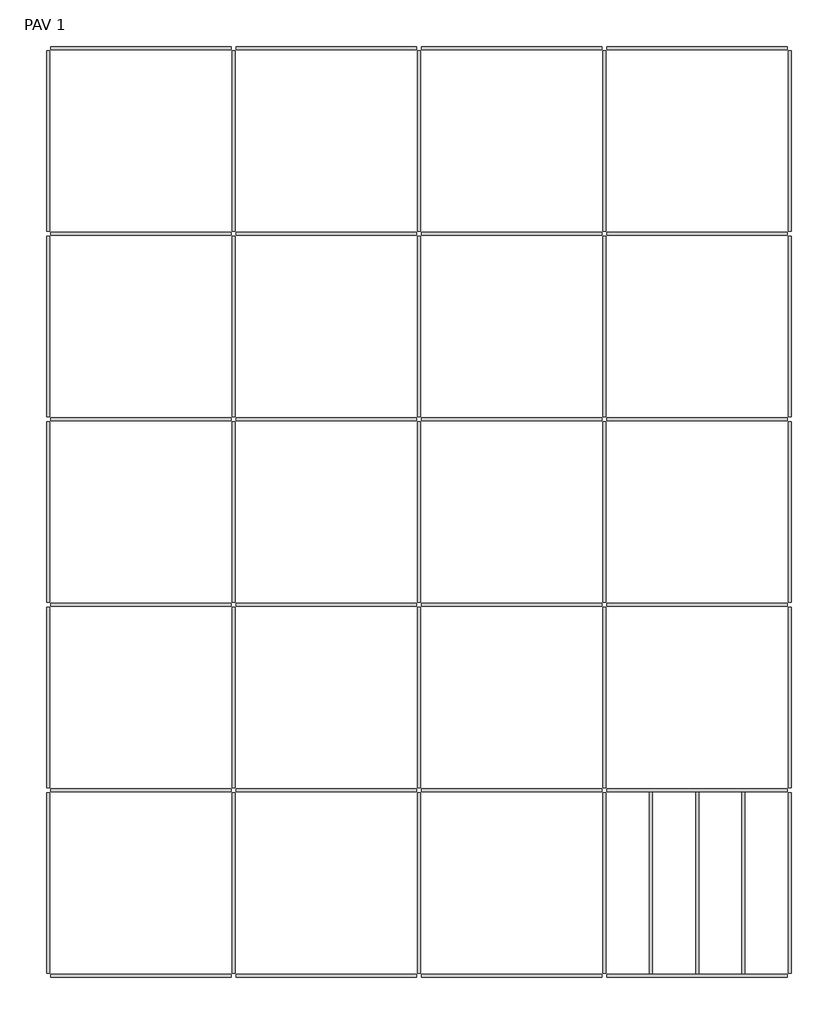
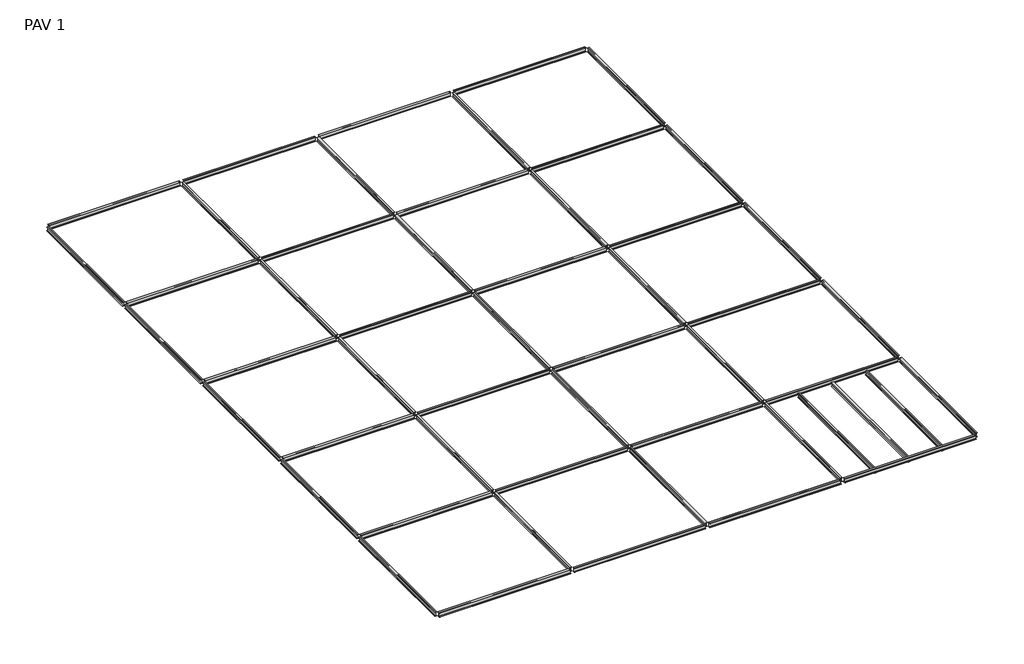
# One storey: 52 beams.
"""IFC4 building model written with IfcOpenShell, lengths in millimetres."""

import ifcopenshell
import ifcopenshell.guid

model = None  # the IFC model being written
_history = None  # IfcOwnerHistory: only IFC2X3 demands one
_inside = {}  # id of a spatial element -> (the spatial element, [elements in it])
_under = {}  # id of a project, library or spatial element -> (it, [spatial elements below it])
_declared = {}  # id of a project -> (the project, [libraries it declares])
_typed = {}  # id of a type object -> (the type object, [elements of that type])
_made_of = {}  # id of a material, layer set ... -> (it, [elements and type objects made of it])


def new_model(schema):
    """Start an empty IFC model of exactly this schema.

    Asked for "IFC4X3", IfcOpenShell would pick the latest addendum, in which some entities
    have other attributes; the version numbers below select the first issue.
    IFC2X3 requires an IfcOwnerHistory on every rooted entity: one is made here for all.
    """
    global model, _history
    if schema == "IFC4X3":
        model = ifcopenshell.file(schema_version=(4, 3, 0, 0))
    else:
        model = ifcopenshell.file(schema=schema)
    _inside.clear()
    _under.clear()
    _declared.clear()
    _typed.clear()
    _made_of.clear()
    _history = None
    if model.schema == "IFC2X3":
        org = make("IfcOrganization", Name="unknown")
        user = make(
            "IfcPersonAndOrganization",
            ThePerson=make("IfcPerson", FamilyName="unknown"),
            TheOrganization=org,
        )
        app = make(
            "IfcApplication",
            ApplicationDeveloper=org,
            Version="unknown",
            ApplicationFullName="unknown",
            ApplicationIdentifier="unknown",
        )
        _history = make(
            "IfcOwnerHistory",
            OwningUser=user,
            OwningApplication=app,
            ChangeAction="ADDED",
            CreationDate=0,
        )
    return model


def make(cls, **values):
    """One entity of the class cls with the attributes given. An attribute that is None is left unset."""
    return model.create_entity(
        cls, **{name: value for name, value in values.items() if value is not None}
    )


def rooted(cls, **values):
    """An entity with a GlobalId (a new one), such as an element, a storey or a relation."""
    return make(cls, GlobalId=ifcopenshell.guid.new(), OwnerHistory=_history, **values)


def si_unit(unit_type, name, prefix=None):
    """IfcSIUnit, for example si_unit("LENGTHUNIT", "METRE", prefix="MILLI")."""
    return make("IfcSIUnit", UnitType=unit_type, Prefix=prefix, Name=name)


def assignment(units):
    """IfcUnitAssignment: the units of a project."""
    return None if units is None else make("IfcUnitAssignment", Units=units)


def point(xyz):
    """IfcCartesianPoint."""
    return None if xyz is None else make("IfcCartesianPoint", Coordinates=xyz)


def direction(xyz):
    """IfcDirection."""
    return None if xyz is None else make("IfcDirection", DirectionRatios=xyz)


def frame(location, z_axis=None, x_axis=None):
    """IfcAxis2Placement3D, a coordinate frame: its origin and axes. An axis left out is left unset."""
    return make(
        "IfcAxis2Placement3D",
        Location=point(location),
        Axis=direction(z_axis),
        RefDirection=direction(x_axis),
    )


def frame_2d(location, x_axis=None):
    """IfcAxis2Placement2D, a coordinate frame in the plane: its origin and x axis."""
    return make(
        "IfcAxis2Placement2D", Location=point(location), RefDirection=direction(x_axis)
    )


def origin():
    """The frame at (0, 0, 0) with its axes left unset."""
    return frame((0.0, 0.0, 0.0))


def place(relative_to, where):
    """IfcLocalPlacement: puts the frame where relative to a parent placement (None: the world)."""
    return make(
        "IfcLocalPlacement", PlacementRelTo=relative_to, RelativePlacement=where
    )


def context(
    kind, dimensions, precision=None, world=None, true_north=None, identifier=None
):
    """IfcGeometricRepresentationContext, for example the 3D "Model" context."""
    return make(
        "IfcGeometricRepresentationContext",
        ContextIdentifier=identifier,
        ContextType=kind,
        CoordinateSpaceDimension=dimensions,
        Precision=precision,
        WorldCoordinateSystem=world,
        TrueNorth=true_north,
    )


def project(units=None, contexts=None):
    """IfcProject with its units and contexts."""
    return rooted(
        "IfcProject",
        Name="project",
        RepresentationContexts=contexts,
        UnitsInContext=assignment(units),
    )


def spatial(cls, under=None, at=None, **own):
    """A site, building, storey or space (cls), placed at a placement, below another one or the project."""
    s = rooted(cls, ObjectPlacement=at, **own)
    if under is not None:
        _under.setdefault(under.id(), (under, []))[1].append(s)
    return s


def polyline(points):
    """IfcPolyline through the points."""
    return make("IfcPolyline", Points=[point(p) for p in points])


def circle_curve(where, radius):
    """IfcCircle in the frame where."""
    return make("IfcCircle", Position=where, Radius=radius)


def trimmed(basis, trim1, trim2, sense, master):
    """IfcTrimmedCurve: the piece of a basis curve between two trims."""
    return make(
        "IfcTrimmedCurve",
        BasisCurve=basis,
        Trim1=trim1,
        Trim2=trim2,
        SenseAgreement=sense,
        MasterRepresentation=master,
    )


def segment(curve, same_sense, transition):
    """IfcCompositeCurveSegment."""
    return make(
        "IfcCompositeCurveSegment",
        Transition=transition,
        SameSense=same_sense,
        ParentCurve=curve,
    )


def composite_curve(segments, self_intersect=None):
    """IfcCompositeCurve: segments joined end to end."""
    return make("IfcCompositeCurve", Segments=segments, SelfIntersect=self_intersect)


def outline(outer, holes=None, kind="AREA"):
    """IfcArbitraryClosedProfileDef: a profile drawn as a closed curve; with holes, ...WithVoids."""
    if holes is None:
        return make("IfcArbitraryClosedProfileDef", ProfileType=kind, OuterCurve=outer)
    return make(
        "IfcArbitraryProfileDefWithVoids",
        ProfileType=kind,
        OuterCurve=outer,
        InnerCurves=holes,
    )


def extrude(swept, where, along, depth):
    """IfcExtrudedAreaSolid: the profile swept, set in the frame where, extruded along a direction by depth."""
    return make(
        "IfcExtrudedAreaSolid",
        SweptArea=swept,
        Position=where,
        ExtrudedDirection=direction(along),
        Depth=depth,
    )


def shape(context_of_items, identifier, shape_type, items):
    """IfcShapeRepresentation: the items that make up one representation, for example the "Body"."""
    return make(
        "IfcShapeRepresentation",
        ContextOfItems=context_of_items,
        RepresentationIdentifier=identifier,
        RepresentationType=shape_type,
        Items=items,
    )


def source(mapping_origin, context_of_items, identifier, shape_type, items):
    """IfcRepresentationMap: a shape defined once, which mapped items show again and again."""
    return make(
        "IfcRepresentationMap",
        MappingOrigin=mapping_origin,
        MappedRepresentation=shape(context_of_items, identifier, shape_type, items),
    )


def transform(
    local_origin,
    x_axis=None,
    y_axis=None,
    z_axis=None,
    scale=None,
    scale2=None,
    scale3=None,
    uniform=True,
):
    """IfcCartesianTransformationOperator3D, or its non-uniform kind. x_axis, y_axis, z_axis: its Axis1, 2, 3."""
    if uniform:
        return make(
            "IfcCartesianTransformationOperator3D",
            Axis1=direction(x_axis),
            Axis2=direction(y_axis),
            LocalOrigin=point(local_origin),
            Scale=scale,
            Axis3=direction(z_axis),
        )
    return make(
        "IfcCartesianTransformationOperator3DnonUniform",
        Axis1=direction(x_axis),
        Axis2=direction(y_axis),
        LocalOrigin=point(local_origin),
        Scale=scale,
        Axis3=direction(z_axis),
        Scale2=scale2,
        Scale3=scale3,
    )


def mapped(mapping_source, mapping_target):
    """IfcMappedItem: shows the shape of a source again, moved by a transform."""
    return make(
        "IfcMappedItem", MappingSource=mapping_source, MappingTarget=mapping_target
    )


def made_of(thing, what):
    """Note that an element or type object is made of a material, layer set ...; save() writes the relation."""
    if what is not None:
        _made_of.setdefault(what.id(), (what, []))[1].append(thing)
    return thing


def element(
    cls,
    number,
    at=None,
    inside=None,
    cuts=None,
    type_object=None,
    material=None,
    context=None,
    identifier="Body",
    shape_type=None,
    held_by="IfcProductDefinitionShape",
    body=None,
    shapes=None,
    **own,
):
    """One element of the class cls, such as IfcWall. Its Tag is "e" and its number.

    at: its placement. inside: the storey or other place that contains it. cuts: it is an
    opening in that element (IfcRelVoidsElement). A single representation is given by context,
    identifier, shape_type and body (its items); several are given by shapes. held_by: the class
    of the entity that holds the representations. save() writes the other relations.
    """
    e = rooted(cls, Tag="e%d" % number, ObjectPlacement=at, **own)
    if body is not None:
        shapes = [shape(context, identifier, shape_type, body)]
    if shapes is not None:
        e.Representation = make(held_by, Representations=shapes)
    if inside is not None:
        _inside.setdefault(inside.id(), (inside, []))[1].append(e)
    if cuts is not None:
        rooted(
            "IfcRelVoidsElement", RelatingBuildingElement=cuts, RelatedOpeningElement=e
        )
    if type_object is not None:
        _typed.setdefault(type_object.id(), (type_object, []))[1].append(e)
    return made_of(e, material)


def aggregate(whole, parts):
    """IfcRelAggregates: a whole, such as a stair, and the parts it consists of."""
    return rooted("IfcRelAggregates", RelatingObject=whole, RelatedObjects=parts)


def save(model, path):
    """Write the relations noted so far, then the file.

    IfcRelAggregates (storeys below a building ...), IfcRelContainedInSpatialStructure (elements
    in a storey), IfcRelDefinesByType, IfcRelAssociatesMaterial and IfcRelDeclares: one each for
    every whole, place, type object, material and project.
    """
    for whole, parts in _under.values():
        aggregate(whole, parts)
    for where, things in _inside.values():
        rooted(
            "IfcRelContainedInSpatialStructure",
            RelatedElements=things,
            RelatingStructure=where,
        )
    for kind, things in _typed.values():
        rooted("IfcRelDefinesByType", RelatedObjects=things, RelatingType=kind)
    for what, things in _made_of.values():
        rooted("IfcRelAssociatesMaterial", RelatedObjects=things, RelatingMaterial=what)
    for by, libraries in _declared.values():
        rooted("IfcRelDeclares", RelatingContext=by, RelatedDefinitions=libraries)
    model.write(path)


def ub_vigas_universais_ub305x165x40_b8b89153(model_context):
    return source(origin(), model_context, "Body", "SweptSolid", [
        extrude(outline(composite_curve([segment(polyline([(82.5, -141.5), (82.5, -151.7), (-82.5, -151.7), (-82.5, -141.5), (-11.9, -141.5)]), True, "CONTINUOUS"), segment(trimmed(circle_curve(frame_2d((-11.9, -132.6)), 8.9), [point((-11.9, -141.5))], [point((-3.0, -132.6))], True, "CARTESIAN"), True, "CONTINUOUS"), segment(polyline([(-3.0, -132.6), (-3.0, 132.6)]), True, "CONTINUOUS"), segment(trimmed(circle_curve(frame_2d((-11.9, 132.6)), 8.9), [point((-3.0, 132.6))], [point((-11.9, 141.5))], True, "CARTESIAN"), True, "CONTINUOUS"), segment(polyline([(-11.9, 141.5), (-82.5, 141.5), (-82.5, 151.7), (82.5, 151.7), (82.5, 141.5), (11.9, 141.5)]), True, "CONTINUOUS"), segment(trimmed(circle_curve(frame_2d((11.9, 132.6)), 8.9), [point((11.9, 141.5))], [point((3.0, 132.6))], True, "CARTESIAN"), True, "CONTINUOUS"), segment(polyline([(3.0, 132.6), (3.0, -132.6)]), True, "CONTINUOUS"), segment(trimmed(circle_curve(frame_2d((11.9, -132.6)), 8.9), [point((3.0, -132.6))], [point((11.9, -141.5))], True, "CARTESIAN"), True, "CONTINUOUS"), segment(polyline([(11.9, -141.5), (82.5, -141.5)]), True, "CONTINUOUS")], self_intersect=False)), frame((-4862.3, 0.0, 0.0), z_axis=(1.0, 0.0, 0.0), x_axis=(0.0, 1.0, 0.0)), (0.0, 0.0, 1.0), 9724.6),
    ])


def ub_vigas_universais_ub305x165x40_08e43834(model_context):
    return source(origin(), model_context, "Body", "SweptSolid", [
        extrude(outline(composite_curve([segment(polyline([(82.5, -141.5), (82.5, -151.7), (-82.5, -151.7), (-82.5, -141.5), (-11.9, -141.5)]), True, "CONTINUOUS"), segment(trimmed(circle_curve(frame_2d((-11.9, -132.6)), 8.9), [point((-11.9, -141.5))], [point((-3.0, -132.6))], True, "CARTESIAN"), True, "CONTINUOUS"), segment(polyline([(-3.0, -132.6), (-3.0, 132.6)]), True, "CONTINUOUS"), segment(trimmed(circle_curve(frame_2d((-11.9, 132.6)), 8.9), [point((-3.0, 132.6))], [point((-11.9, 141.5))], True, "CARTESIAN"), True, "CONTINUOUS"), segment(polyline([(-11.9, 141.5), (-82.5, 141.5), (-82.5, 151.7), (82.5, 151.7), (82.5, 141.5), (11.9, 141.5)]), True, "CONTINUOUS"), segment(trimmed(circle_curve(frame_2d((11.9, 132.6)), 8.9), [point((11.9, 141.5))], [point((3.0, 132.6))], True, "CARTESIAN"), True, "CONTINUOUS"), segment(polyline([(3.0, 132.6), (3.0, -132.6)]), True, "CONTINUOUS"), segment(trimmed(circle_curve(frame_2d((11.9, -132.6)), 8.9), [point((3.0, -132.6))], [point((11.9, -141.5))], True, "CARTESIAN"), True, "CONTINUOUS"), segment(polyline([(11.9, -141.5), (82.5, -141.5)]), True, "CONTINUOUS")], self_intersect=False)), frame((-4904.8, 0.0, 0.0), z_axis=(1.0, 0.0, 0.0), x_axis=(0.0, 1.0, 0.0)), (0.0, 0.0, 1.0), 9809.6),
    ])


model = new_model("IFC4")

# Units and contexts
model_context = context("Model", 3, world=origin())
ifc_project = project(units=[si_unit("LENGTHUNIT", "METRE", prefix="MILLI")], contexts=[model_context])

# Site, building, storey
site = spatial("IfcSite", under=ifc_project)
building = spatial("IfcBuilding", under=site)
storey = spatial("IfcBuildingStorey", under=building, Name="PAV 1", Elevation=43565.0)

# Beams
placement = place(None, origin())
ub_vigas_universais_ub305x165x40_shape = ub_vigas_universais_ub305x165x40_b8b89153(model_context)
element("IfcBeam", 1, ObjectType="UB-Vigas universais : UB305x165x40", at=placement, inside=storey, context=model_context, shape_type="MappedRepresentation", body=[
    mapped(ub_vigas_universais_ub305x165x40_shape, transform((-11703.8168708, -32103.5623634, 43578.3), x_axis=(0.0, 1.0, 0.0), y_axis=(-1.0, 0.0, 0.0), z_axis=(0.0, 0.0, 1.0))),
])
element("IfcBeam", 2, ObjectType="UB-Vigas universais : UB305x165x40", at=placement, inside=storey, context=model_context, shape_type="MappedRepresentation", body=[
    mapped(ub_vigas_universais_ub305x165x40_shape, transform((-11703.8168708, -22103.5623634, 43578.3), x_axis=(0.0, 1.0, 0.0), y_axis=(-1.0, 0.0, 0.0), z_axis=(0.0, 0.0, 1.0))),
])
element("IfcBeam", 3, ObjectType="UB-Vigas universais : UB305x165x40", at=placement, inside=storey, context=model_context, shape_type="MappedRepresentation", body=[
    mapped(ub_vigas_universais_ub305x165x40_shape, transform((-11703.8168708, -12103.5623634, 43578.3), x_axis=(0.0, 1.0, 0.0), y_axis=(-1.0, 0.0, 0.0), z_axis=(0.0, 0.0, 1.0))),
])
element("IfcBeam", 4, ObjectType="UB-Vigas universais : UB305x165x40", at=placement, inside=storey, context=model_context, shape_type="MappedRepresentation", body=[
    mapped(ub_vigas_universais_ub305x165x40_shape, transform((-11703.8168708, -2103.5623634, 43578.3), x_axis=(0.0, 1.0, 0.0), y_axis=(-1.0, 0.0, 0.0), z_axis=(0.0, 0.0, 1.0))),
])
element("IfcBeam", 5, ObjectType="UB-Vigas universais : UB305x165x40", at=placement, inside=storey, context=model_context, shape_type="MappedRepresentation", body=[
    mapped(ub_vigas_universais_ub305x165x40_shape, transform((-11703.8168708, 7896.4376366, 43578.3), x_axis=(0.0, 1.0, 0.0), y_axis=(-1.0, 0.0, 0.0), z_axis=(0.0, 0.0, 1.0))),
])
element("IfcBeam", 6, ObjectType="UB-Vigas universais : UB305x165x40", at=placement, inside=storey, context=model_context, shape_type="MappedRepresentation", body=[
    mapped(ub_vigas_universais_ub305x165x40_shape, transform((-1703.8168708, 7896.4376366, 43578.3), x_axis=(0.0, -1.0, 0.0), y_axis=(1.0, 0.0, 0.0), z_axis=(0.0, 0.0, 1.0))),
])
element("IfcBeam", 7, ObjectType="UB-Vigas universais : UB305x165x40", at=placement, inside=storey, context=model_context, shape_type="MappedRepresentation", body=[
    mapped(ub_vigas_universais_ub305x165x40_shape, transform((-1703.8168708, -2103.5623634, 43578.3), x_axis=(0.0, -1.0, 0.0), y_axis=(1.0, 0.0, 0.0), z_axis=(0.0, 0.0, 1.0))),
])
element("IfcBeam", 8, ObjectType="UB-Vigas universais : UB305x165x40", at=placement, inside=storey, context=model_context, shape_type="MappedRepresentation", body=[
    mapped(ub_vigas_universais_ub305x165x40_shape, transform((-1703.8168708, -12103.5623634, 43578.3), x_axis=(0.0, -1.0, 0.0), y_axis=(1.0, 0.0, 0.0), z_axis=(0.0, 0.0, 1.0))),
])
element("IfcBeam", 9, ObjectType="UB-Vigas universais : UB305x165x40", at=placement, inside=storey, context=model_context, shape_type="MappedRepresentation", body=[
    mapped(ub_vigas_universais_ub305x165x40_shape, transform((-1703.8168708, -22103.5623634, 43578.3), x_axis=(0.0, -1.0, 0.0), y_axis=(1.0, 0.0, 0.0), z_axis=(0.0, 0.0, 1.0))),
])
element("IfcBeam", 10, ObjectType="UB-Vigas universais : UB305x165x40", at=placement, inside=storey, context=model_context, shape_type="MappedRepresentation", body=[
    mapped(ub_vigas_universais_ub305x165x40_shape, transform((-1703.8168708, -32103.5623634, 43578.3), x_axis=(0.0, -1.0, 0.0), y_axis=(1.0, 0.0, 0.0), z_axis=(0.0, 0.0, 1.0))),
])
element("IfcBeam", 11, ObjectType="UB-Vigas universais : UB305x165x40", at=placement, inside=storey, context=model_context, shape_type="MappedRepresentation", body=[
    mapped(ub_vigas_universais_ub305x165x40_shape, transform((8296.1831292, 7896.4376366, 43578.3), x_axis=(0.0, -1.0, 0.0), y_axis=(1.0, 0.0, 0.0), z_axis=(0.0, 0.0, 1.0))),
])
element("IfcBeam", 12, ObjectType="UB-Vigas universais : UB305x165x40", at=placement, inside=storey, context=model_context, shape_type="MappedRepresentation", body=[
    mapped(ub_vigas_universais_ub305x165x40_shape, transform((8296.1831292, -2103.5623634, 43578.3), x_axis=(0.0, -1.0, 0.0), y_axis=(1.0, 0.0, 0.0), z_axis=(0.0, 0.0, 1.0))),
])
element("IfcBeam", 13, ObjectType="UB-Vigas universais : UB305x165x40", at=placement, inside=storey, context=model_context, shape_type="MappedRepresentation", body=[
    mapped(ub_vigas_universais_ub305x165x40_shape, transform((8296.1831292, -12103.5623634, 43578.3), x_axis=(0.0, -1.0, 0.0), y_axis=(1.0, 0.0, 0.0), z_axis=(0.0, 0.0, 1.0))),
])
element("IfcBeam", 14, ObjectType="UB-Vigas universais : UB305x165x40", at=placement, inside=storey, context=model_context, shape_type="MappedRepresentation", body=[
    mapped(ub_vigas_universais_ub305x165x40_shape, transform((8296.1831292, -22103.5623634, 43578.3), x_axis=(0.0, -1.0, 0.0), y_axis=(1.0, 0.0, 0.0), z_axis=(0.0, 0.0, 1.0))),
])
element("IfcBeam", 15, ObjectType="UB-Vigas universais : UB305x165x40", at=placement, inside=storey, context=model_context, shape_type="MappedRepresentation", body=[
    mapped(ub_vigas_universais_ub305x165x40_shape, transform((8296.1831292, -32103.5623634, 43578.3), x_axis=(0.0, -1.0, 0.0), y_axis=(1.0, 0.0, 0.0), z_axis=(0.0, 0.0, 1.0))),
])
element("IfcBeam", 16, ObjectType="UB-Vigas universais : UB305x165x40", at=placement, inside=storey, context=model_context, shape_type="MappedRepresentation", body=[
    mapped(ub_vigas_universais_ub305x165x40_shape, transform((18296.1831292, 7896.4376366, 43578.3), x_axis=(0.0, -1.0, 0.0), y_axis=(1.0, 0.0, 0.0), z_axis=(0.0, 0.0, 1.0))),
])
element("IfcBeam", 17, ObjectType="UB-Vigas universais : UB305x165x40", at=placement, inside=storey, context=model_context, shape_type="MappedRepresentation", body=[
    mapped(ub_vigas_universais_ub305x165x40_shape, transform((18296.1831292, -2103.5623634, 43578.3), x_axis=(0.0, -1.0, 0.0), y_axis=(1.0, 0.0, 0.0), z_axis=(0.0, 0.0, 1.0))),
])
element("IfcBeam", 18, ObjectType="UB-Vigas universais : UB305x165x40", at=placement, inside=storey, context=model_context, shape_type="MappedRepresentation", body=[
    mapped(ub_vigas_universais_ub305x165x40_shape, transform((18296.1831292, -12103.5623634, 43578.3), x_axis=(0.0, -1.0, 0.0), y_axis=(1.0, 0.0, 0.0), z_axis=(0.0, 0.0, 1.0))),
])
element("IfcBeam", 19, ObjectType="UB-Vigas universais : UB305x165x40", at=placement, inside=storey, context=model_context, shape_type="MappedRepresentation", body=[
    mapped(ub_vigas_universais_ub305x165x40_shape, transform((18296.1831292, -22103.5623634, 43578.3), x_axis=(0.0, -1.0, 0.0), y_axis=(1.0, 0.0, 0.0), z_axis=(0.0, 0.0, 1.0))),
])
element("IfcBeam", 20, ObjectType="UB-Vigas universais : UB305x165x40", at=placement, inside=storey, context=model_context, shape_type="MappedRepresentation", body=[
    mapped(ub_vigas_universais_ub305x165x40_shape, transform((18296.1831292, -32103.5623634, 43578.3), x_axis=(0.0, -1.0, 0.0), y_axis=(1.0, 0.0, 0.0), z_axis=(0.0, 0.0, 1.0))),
])
element("IfcBeam", 21, ObjectType="UB-Vigas universais : UB305x165x40", at=placement, inside=storey, context=model_context, shape_type="MappedRepresentation", body=[
    mapped(ub_vigas_universais_ub305x165x40_shape, transform((-6703.8168708, 12896.4376366, 43578.3), x_axis=(1.0, 0.0, 0.0), y_axis=(0.0, 1.0, 0.0), z_axis=(0.0, 0.0, 1.0))),
])
element("IfcBeam", 22, ObjectType="UB-Vigas universais : UB305x165x40", at=placement, inside=storey, context=model_context, shape_type="MappedRepresentation", body=[
    mapped(ub_vigas_universais_ub305x165x40_shape, transform((3296.1831292, 12896.4376366, 43578.3), x_axis=(1.0, 0.0, 0.0), y_axis=(0.0, 1.0, 0.0), z_axis=(0.0, 0.0, 1.0))),
])
element("IfcBeam", 23, ObjectType="UB-Vigas universais : UB305x165x40", at=placement, inside=storey, context=model_context, shape_type="MappedRepresentation", body=[
    mapped(ub_vigas_universais_ub305x165x40_shape, transform((13296.1831292, 12896.4376366, 43578.3), x_axis=(1.0, 0.0, 0.0), y_axis=(0.0, 1.0, 0.0), z_axis=(0.0, 0.0, 1.0))),
])
element("IfcBeam", 24, ObjectType="UB-Vigas universais : UB305x165x40", at=placement, inside=storey, context=model_context, shape_type="MappedRepresentation", body=[
    mapped(ub_vigas_universais_ub305x165x40_shape, transform((23296.1831292, 12896.4376366, 43578.3), x_axis=(1.0, 0.0, 0.0), y_axis=(0.0, 1.0, 0.0), z_axis=(0.0, 0.0, 1.0))),
])
element("IfcBeam", 25, ObjectType="UB-Vigas universais : UB305x165x40", at=placement, inside=storey, context=model_context, shape_type="MappedRepresentation", body=[
    mapped(ub_vigas_universais_ub305x165x40_shape, transform((23296.1831292, 2896.4376366, 43578.3), x_axis=(-1.0, 0.0, 0.0), y_axis=(0.0, -1.0, 0.0), z_axis=(0.0, 0.0, 1.0))),
])
element("IfcBeam", 26, ObjectType="UB-Vigas universais : UB305x165x40", at=placement, inside=storey, context=model_context, shape_type="MappedRepresentation", body=[
    mapped(ub_vigas_universais_ub305x165x40_shape, transform((13296.1831292, 2896.4376366, 43578.3), x_axis=(-1.0, 0.0, 0.0), y_axis=(0.0, -1.0, 0.0), z_axis=(0.0, 0.0, 1.0))),
])
element("IfcBeam", 27, ObjectType="UB-Vigas universais : UB305x165x40", at=placement, inside=storey, context=model_context, shape_type="MappedRepresentation", body=[
    mapped(ub_vigas_universais_ub305x165x40_shape, transform((3296.1831292, 2896.4376366, 43578.3), x_axis=(-1.0, 0.0, 0.0), y_axis=(0.0, -1.0, 0.0), z_axis=(0.0, 0.0, 1.0))),
])
element("IfcBeam", 28, ObjectType="UB-Vigas universais : UB305x165x40", at=placement, inside=storey, context=model_context, shape_type="MappedRepresentation", body=[
    mapped(ub_vigas_universais_ub305x165x40_shape, transform((-6703.8168708, 2896.4376366, 43578.3), x_axis=(-1.0, 0.0, 0.0), y_axis=(0.0, -1.0, 0.0), z_axis=(0.0, 0.0, 1.0))),
])
element("IfcBeam", 29, ObjectType="UB-Vigas universais : UB305x165x40", at=placement, inside=storey, context=model_context, shape_type="MappedRepresentation", body=[
    mapped(ub_vigas_universais_ub305x165x40_shape, transform((23296.1831292, -7103.5623634, 43578.3), x_axis=(-1.0, 0.0, 0.0), y_axis=(0.0, -1.0, 0.0), z_axis=(0.0, 0.0, 1.0))),
])
element("IfcBeam", 30, ObjectType="UB-Vigas universais : UB305x165x40", at=placement, inside=storey, context=model_context, shape_type="MappedRepresentation", body=[
    mapped(ub_vigas_universais_ub305x165x40_shape, transform((13296.1831292, -7103.5623634, 43578.3), x_axis=(-1.0, 0.0, 0.0), y_axis=(0.0, -1.0, 0.0), z_axis=(0.0, 0.0, 1.0))),
])
element("IfcBeam", 31, ObjectType="UB-Vigas universais : UB305x165x40", at=placement, inside=storey, context=model_context, shape_type="MappedRepresentation", body=[
    mapped(ub_vigas_universais_ub305x165x40_shape, transform((3296.1831292, -7103.5623634, 43578.3), x_axis=(-1.0, 0.0, 0.0), y_axis=(0.0, -1.0, 0.0), z_axis=(0.0, 0.0, 1.0))),
])
element("IfcBeam", 32, ObjectType="UB-Vigas universais : UB305x165x40", at=placement, inside=storey, context=model_context, shape_type="MappedRepresentation", body=[
    mapped(ub_vigas_universais_ub305x165x40_shape, transform((-6703.8168708, -7103.5623634, 43578.3), x_axis=(-1.0, 0.0, 0.0), y_axis=(0.0, -1.0, 0.0), z_axis=(0.0, 0.0, 1.0))),
])
element("IfcBeam", 33, ObjectType="UB-Vigas universais : UB305x165x40", at=placement, inside=storey, context=model_context, shape_type="MappedRepresentation", body=[
    mapped(ub_vigas_universais_ub305x165x40_shape, transform((23296.1831292, -17103.5623634, 43578.3), x_axis=(-1.0, 0.0, 0.0), y_axis=(0.0, -1.0, 0.0), z_axis=(0.0, 0.0, 1.0))),
])
element("IfcBeam", 34, ObjectType="UB-Vigas universais : UB305x165x40", at=placement, inside=storey, context=model_context, shape_type="MappedRepresentation", body=[
    mapped(ub_vigas_universais_ub305x165x40_shape, transform((13296.1831292, -17103.5623634, 43578.3), x_axis=(-1.0, 0.0, 0.0), y_axis=(0.0, -1.0, 0.0), z_axis=(0.0, 0.0, 1.0))),
])
element("IfcBeam", 35, ObjectType="UB-Vigas universais : UB305x165x40", at=placement, inside=storey, context=model_context, shape_type="MappedRepresentation", body=[
    mapped(ub_vigas_universais_ub305x165x40_shape, transform((3296.1831292, -17103.5623634, 43578.3), x_axis=(-1.0, 0.0, 0.0), y_axis=(0.0, -1.0, 0.0), z_axis=(0.0, 0.0, 1.0))),
])
element("IfcBeam", 36, ObjectType="UB-Vigas universais : UB305x165x40", at=placement, inside=storey, context=model_context, shape_type="MappedRepresentation", body=[
    mapped(ub_vigas_universais_ub305x165x40_shape, transform((-6703.8168708, -17103.5623634, 43578.3), x_axis=(-1.0, 0.0, 0.0), y_axis=(0.0, -1.0, 0.0), z_axis=(0.0, 0.0, 1.0))),
])
element("IfcBeam", 37, ObjectType="UB-Vigas universais : UB305x165x40", at=placement, inside=storey, context=model_context, shape_type="MappedRepresentation", body=[
    mapped(ub_vigas_universais_ub305x165x40_shape, transform((23296.1831292, -27103.5623634, 43578.3), x_axis=(-1.0, 0.0, 0.0), y_axis=(0.0, -1.0, 0.0), z_axis=(0.0, 0.0, 1.0))),
])
element("IfcBeam", 38, ObjectType="UB-Vigas universais : UB305x165x40", at=placement, inside=storey, context=model_context, shape_type="MappedRepresentation", body=[
    mapped(ub_vigas_universais_ub305x165x40_shape, transform((13296.1831292, -27103.5623634, 43578.3), x_axis=(-1.0, 0.0, 0.0), y_axis=(0.0, -1.0, 0.0), z_axis=(0.0, 0.0, 1.0))),
])
element("IfcBeam", 39, ObjectType="UB-Vigas universais : UB305x165x40", at=placement, inside=storey, context=model_context, shape_type="MappedRepresentation", body=[
    mapped(ub_vigas_universais_ub305x165x40_shape, transform((3296.1831292, -27103.5623634, 43578.3), x_axis=(-1.0, 0.0, 0.0), y_axis=(0.0, -1.0, 0.0), z_axis=(0.0, 0.0, 1.0))),
])
element("IfcBeam", 40, ObjectType="UB-Vigas universais : UB305x165x40", at=placement, inside=storey, context=model_context, shape_type="MappedRepresentation", body=[
    mapped(ub_vigas_universais_ub305x165x40_shape, transform((-6703.8168708, -27103.5623634, 43578.3), x_axis=(-1.0, 0.0, 0.0), y_axis=(0.0, -1.0, 0.0), z_axis=(0.0, 0.0, 1.0))),
])
element("IfcBeam", 41, ObjectType="UB-Vigas universais : UB305x165x40", at=placement, inside=storey, context=model_context, shape_type="MappedRepresentation", body=[
    mapped(ub_vigas_universais_ub305x165x40_shape, transform((23296.1831292, -37103.5623634, 43578.3), x_axis=(-1.0, 0.0, 0.0), y_axis=(0.0, -1.0, 0.0), z_axis=(0.0, 0.0, 1.0))),
])
element("IfcBeam", 42, ObjectType="UB-Vigas universais : UB305x165x40", at=placement, inside=storey, context=model_context, shape_type="MappedRepresentation", body=[
    mapped(ub_vigas_universais_ub305x165x40_shape, transform((13296.1831292, -37103.5623634, 43578.3), x_axis=(-1.0, 0.0, 0.0), y_axis=(0.0, -1.0, 0.0), z_axis=(0.0, 0.0, 1.0))),
])
element("IfcBeam", 43, ObjectType="UB-Vigas universais : UB305x165x40", at=placement, inside=storey, context=model_context, shape_type="MappedRepresentation", body=[
    mapped(ub_vigas_universais_ub305x165x40_shape, transform((3296.1831292, -37103.5623634, 43578.3), x_axis=(-1.0, 0.0, 0.0), y_axis=(0.0, -1.0, 0.0), z_axis=(0.0, 0.0, 1.0))),
])
element("IfcBeam", 44, ObjectType="UB-Vigas universais : UB305x165x40", at=placement, inside=storey, context=model_context, shape_type="MappedRepresentation", body=[
    mapped(ub_vigas_universais_ub305x165x40_shape, transform((-6703.8168708, -37103.5623634, 43578.3), x_axis=(-1.0, 0.0, 0.0), y_axis=(0.0, -1.0, 0.0), z_axis=(0.0, 0.0, 1.0))),
])
element("IfcBeam", 45, ObjectType="UB-Vigas universais : UB305x165x40", at=placement, inside=storey, context=model_context, shape_type="MappedRepresentation", body=[
    mapped(ub_vigas_universais_ub305x165x40_shape, transform((28296.1831292, -32103.5623634, 43578.3), x_axis=(0.0, 1.0, 0.0), y_axis=(-1.0, 0.0, 0.0), z_axis=(0.0, 0.0, 1.0))),
])
element("IfcBeam", 46, ObjectType="UB-Vigas universais : UB305x165x40", at=placement, inside=storey, context=model_context, shape_type="MappedRepresentation", body=[
    mapped(ub_vigas_universais_ub305x165x40_shape, transform((28296.1831292, -22103.5623634, 43578.3), x_axis=(0.0, 1.0, 0.0), y_axis=(-1.0, 0.0, 0.0), z_axis=(0.0, 0.0, 1.0))),
])
element("IfcBeam", 47, ObjectType="UB-Vigas universais : UB305x165x40", at=placement, inside=storey, context=model_context, shape_type="MappedRepresentation", body=[
    mapped(ub_vigas_universais_ub305x165x40_shape, transform((28296.1831292, -12103.5623634, 43578.3), x_axis=(0.0, 1.0, 0.0), y_axis=(-1.0, 0.0, 0.0), z_axis=(0.0, 0.0, 1.0))),
])
element("IfcBeam", 48, ObjectType="UB-Vigas universais : UB305x165x40", at=placement, inside=storey, context=model_context, shape_type="MappedRepresentation", body=[
    mapped(ub_vigas_universais_ub305x165x40_shape, transform((28296.1831292, -2103.5623634, 43578.3), x_axis=(0.0, 1.0, 0.0), y_axis=(-1.0, 0.0, 0.0), z_axis=(0.0, 0.0, 1.0))),
])
element("IfcBeam", 49, ObjectType="UB-Vigas universais : UB305x165x40", at=placement, inside=storey, context=model_context, shape_type="MappedRepresentation", body=[
    mapped(ub_vigas_universais_ub305x165x40_shape, transform((28296.1831292, 7896.4376366, 43578.3), x_axis=(0.0, 1.0, 0.0), y_axis=(-1.0, 0.0, 0.0), z_axis=(0.0, 0.0, 1.0))),
])
ub_vigas_universais_ub305x165x40_2_shape = ub_vigas_universais_ub305x165x40_08e43834(model_context)
element("IfcBeam", 50, ObjectType="UB-Vigas universais : UB305x165x40", at=placement, inside=storey, context=model_context, shape_type="MappedRepresentation", body=[
    mapped(ub_vigas_universais_ub305x165x40_2_shape, transform((20796.1831292, -32103.5623634, 43413.3), x_axis=(0.0, 1.0, 0.0), y_axis=(-1.0, 0.0, 0.0), z_axis=(0.0, 0.0, 1.0))),
])
element("IfcBeam", 51, ObjectType="UB-Vigas universais : UB305x165x40", at=placement, inside=storey, context=model_context, shape_type="MappedRepresentation", body=[
    mapped(ub_vigas_universais_ub305x165x40_2_shape, transform((23296.1831292, -32103.5623634, 43413.3), x_axis=(0.0, 1.0, 0.0), y_axis=(-1.0, 0.0, 0.0), z_axis=(0.0, 0.0, 1.0))),
])
element("IfcBeam", 52, ObjectType="UB-Vigas universais : UB305x165x40", at=placement, inside=storey, context=model_context, shape_type="MappedRepresentation", body=[
    mapped(ub_vigas_universais_ub305x165x40_2_shape, transform((25796.1831292, -32103.5623634, 43413.3), x_axis=(0.0, 1.0, 0.0), y_axis=(-1.0, 0.0, 0.0), z_axis=(0.0, 0.0, 1.0))),
])

save(model, "model.ifc")

# Revit data of these elements
# Type "UB-Vigas universais : UB305x165x40"
#   Section Name Key = "UB305X165X40"
#   Width = 16.5 cm
#   Web Thickness = 0.6 cm
#   Web Fillet = 0.89 cm
#   Warping Constant = 164000.0 cm⁶
#   Torsional Moment of Inertia = 14.70 cm⁴
#   Section Area = 51.3 cm²
#   Plastic Modulus weak axis = 142.0 cm³
#   Plastic Modulus strong axis = 623.0 cm³
#   Nominal Weight = 40.2999 kgf/m
#   Moment of Inertia weak axis = 764.00 cm⁴
#   Moment of Inertia strong axis = 8503.00 cm⁴
#   Height = 30.34 cm
#   Flange Thickness = 1.02 cm
#   Elastic Modulus weak axis = 92.6 cm³
#   Elastic Modulus strong axis = 560.0 cm³
#   Centroid Vertical = 15.17 cm
#   Centroid Horizontal = 8.25 cm
#   Length [instance default] = 1.50 m
#   Structural Material [instance default] = Metal - Aço 43-275
#   Type Comments = ""
#   Assembly Code = ""
# Elements 1, 2, 3, 4, 5, 6, 7, 8, 9, 10, 11, 12, 13, 14, 15, 16, 17, 18, 19, 20, 21, 22, 23, 24, 25, 26, 27, 28, 29, 30, 31, 32, 33, 34, 35, 36, 37, 38, 39, 40, 41, 42, 43, 44, 45, 46, 47, 48, 49 (IfcBeam, "UB-Vigas universais : UB305x165x40")
#   Comments = ""
#   Structural Material = Metal - Aço 43-275
#   Phase Created = Construção nova
#   Materials on its faces: "Metal - Aço 43-275"
# Elements 50, 51, 52 (IfcBeam, "UB-Vigas universais : UB305x165x40")
#   Structural Material = Metal - Aço 43-275
#   Phase Created = Construção nova
#   Materials on its faces: "Metal - Aço 43-275"
# Materials
#   "Metal - Aço 43-275": class "Metal", colour RGB 247 247 247, transparency 0, Cost = 0
